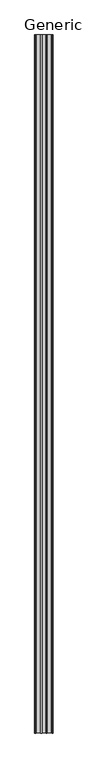
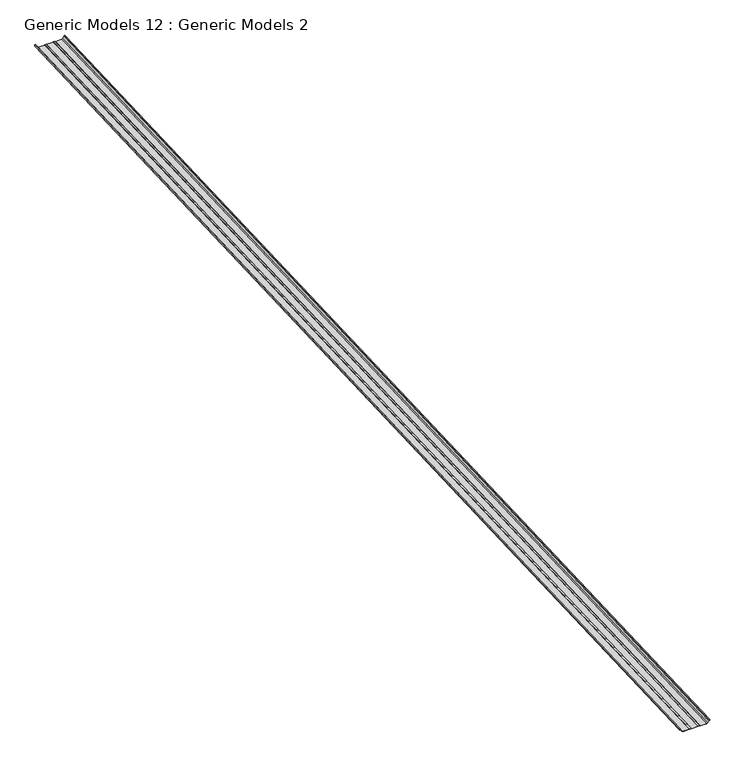
"""IFC4 building model written with IfcOpenShell, lengths in millimetres: proxy geometry, Generic Models 12 : Generic Models 2."""

from ifc_helpers import new_model, si_unit, frame, origin, place, context, project, spatial, polyline, outline, extrude, source, transform, mapped, element, save


def generic_models_12_generic_models_2_a49e82a3(model_context):
    return source(origin(), model_context, "Body", "SweptSolid", [
        extrude(outline(polyline([(-23.4855078, -1e-07), (10.581726, 0.0), (10.5173649, 14.4944601), (12.1048492, 14.5015091), (12.1762907, -1.5875001), (-25.0659743, -1.5875001), (-25.1976147, 28.058605), (-80.3528451, 50.0600224), (-99.2378645, 83.8258891), (-100.1331933, 285.4586309), (-93.2338635, 289.4828908), (-93.4564582, 339.6123832), (-100.3912533, 343.5750931), (-101.2817013, 544.1086597), (-94.3823715, 548.1329196), (-94.6049662, 598.262412), (-101.5397613, 602.2251219), (-102.4274889, 802.146015), (-83.7787769, 834.7818777), (-28.8863391, 857.2438025), (-29.0181014, 886.9173666), (9.8623855, 887.0115215), (10.0083155, 885.4243702), (-27.4235537, 885.3337233), (-27.2941, 856.180078), (-82.6716399, 833.51965), (-100.8381158, 801.7277163), (-99.9563468, 603.1487219), (-93.0215518, 599.1860121), (-92.7908174, 547.2234315), (-99.6901472, 543.1991716), (-98.8078387, 344.4986931), (-91.8730437, 340.5359833), (-91.6423094, 288.5734027), (-98.5416391, 284.5491428), (-97.6522007, 84.2429512), (-79.2420015, 51.326049), (-23.6148849, 29.1363962), (-23.4855078, -1e-07)])), frame((666578.9705225, -569967.8994802, 8837.9605844), z_axis=(0.0, 0.9991330730923522, 0.04163054471217685), x_axis=(-0.00444035025207142, -0.04163013430145772, 0.9991232232350931)), (0.0, 0.0, 1.0), 33406.7702703),
    ])


if __name__ == "__main__":
    model = new_model("IFC4")
    model_context = context("Model", 3, world=origin())
    ifc_project = project(units=[si_unit("LENGTHUNIT", "METRE", prefix="MILLI")], contexts=[model_context])
    site = spatial("IfcSite", under=ifc_project)
    building = spatial("IfcBuilding", under=site)
    placement = place(None, origin())
    generic_models_12_generic_models_2_shape = generic_models_12_generic_models_2_a49e82a3(model_context)
    element("IfcBuildingElementProxy", 1, Name="Generic Models 12 : Generic Models 2", ObjectType="Generic Models 12 : Generic Models 2", at=placement, inside=building, context=model_context, shape_type="MappedRepresentation", body=[
        mapped(generic_models_12_generic_models_2_shape, transform((0.0, 0.0, 0.0), x_axis=(1.0, 0.0, 0.0), y_axis=(0.0, 1.0, 0.0), z_axis=(0.0, 0.0, 1.0))),
    ])
    save(model, "model.ifc")

# Revit data of these elements
# Element 1 (IfcBuildingElementProxy, "Generic Models 12 : Generic Models 2")
#   Materials on its faces: "STRUCTURAL STANDING SEAM SHEET METAL ROOFING - DOUBLE-LOK - COLOR T.B.D."
# Materials
#   "STRUCTURAL STANDING SEAM SHEET METAL ROOFING - DOUBLE-LOK - COLOR T.B.D.": class "Generic", colour RGB 192 192 192, transparency 0, Cost = 0
